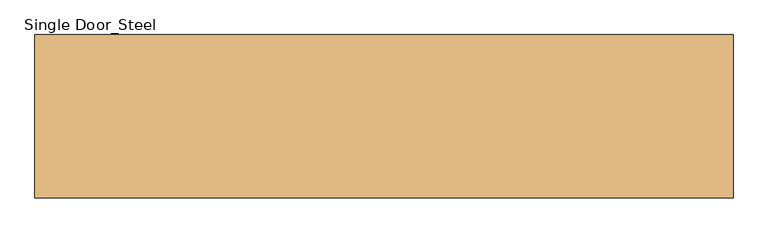
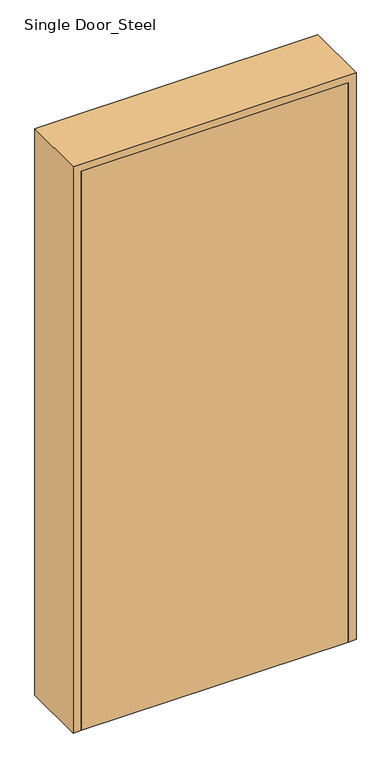
"""IFC4 building model written with IfcOpenShell, lengths in millimetres: door geometry, Single Door_Steel : H_DR_AR B12_Door_Single_W1100xH2280_FR 1.0H_FSD-1."""

from ifc_helpers import new_model, si_unit, origin, origin_with_axes, place, context, project, spatial, polyline, outline, extrude, faceted_brep, source, transform, mapped, element, save


def single_door_steel_8b0dfbf3(model_context):
    return source(origin(), model_context, "Body", "SolidModel", [
        extrude(outline(polyline([(505.0, -125.0), (-505.0, -125.0), (-505.0, -85.0), (505.0, -85.0), (505.0, -125.0)])), origin_with_axes(), (0.0, 0.0, 1.0), 2235.0),
        faceted_brep([(505.0, -125.0, 0.0), (505.0, -85.0, 0.0), (485.0, -85.0, 0.0), (485.0, 85.0, 0.0), (505.0, 85.0, 0.0), (505.0, 125.0, 0.0), (535.0, 125.0, 0.0), (535.0, -125.0, 0.0), (-505.0, -125.0, 0.0), (-535.0, -125.0, 0.0), (-535.0, 125.0, 0.0), (-505.0, 125.0, 0.0), (-505.0, 85.0, 0.0), (-485.0, 85.0, 0.0), (-485.0, -85.0, 0.0), (-505.0, -85.0, 0.0), (535.0, -125.0, 2265.0), (-535.0, -125.0, 2265.0), (-505.0, -125.0, 2235.0), (505.0, -125.0, 2235.0), (535.0, 125.0, 2265.0), (505.0, 125.0, 2235.0), (-505.0, 125.0, 2235.0), (-535.0, 125.0, 2265.0), (505.0, 85.0, 2235.0), (485.0, 85.0, 2215.0), (-485.0, 85.0, 2215.0), (-505.0, 85.0, 2235.0), (485.0, -85.0, 2215.0), (505.0, -85.0, 2235.0), (-505.0, -85.0, 2235.0), (-485.0, -85.0, 2215.0)], [[[0, 1, 2, 3, 4, 5, 6, 7]], [[8, 9, 10, 11, 12, 13, 14, 15]], [[7, 16, 17, 9, 8, 18, 19, 0]], [[6, 20, 16, 7]], [[5, 21, 22, 11, 10, 23, 20, 6]], [[4, 24, 21, 5]], [[3, 25, 26, 13, 12, 27, 24, 4]], [[2, 28, 25, 3]], [[1, 29, 30, 15, 14, 31, 28, 2]], [[0, 19, 29, 1]], [[18, 8, 15, 30]], [[23, 10, 9, 17]], [[27, 12, 11, 22]], [[31, 14, 13, 26]], [[20, 23, 17, 16]], [[24, 27, 22, 21]], [[28, 31, 26, 25]], [[19, 18, 30, 29]]]),
    ])


if __name__ == "__main__":
    model = new_model("IFC4")
    model_context = context("Model", 3, world=origin())
    ifc_project = project(units=[si_unit("LENGTHUNIT", "METRE", prefix="MILLI")], contexts=[model_context])
    site = spatial("IfcSite", under=ifc_project)
    building = spatial("IfcBuilding", under=site)
    placement = place(None, origin())
    single_door_steel_shape = single_door_steel_8b0dfbf3(model_context)
    element("IfcDoor", 1, ObjectType="Single Door_Steel : H_DR_AR B12_Door_Single_W1100xH2280_FR 1.0H_FSD-1", at=placement, inside=building, context=model_context, shape_type="MappedRepresentation", body=[
        mapped(single_door_steel_shape, transform((0.0, 0.0, 0.0), x_axis=(1.0, 0.0, 0.0), y_axis=(0.0, 1.0, 0.0), z_axis=(0.0, 0.0, 1.0))),
    ])
    save(model, "model.ifc")

# Revit data of these elements
# Type "Single Door_Steel : H_DR_AR B12_Door_Single_W1100xH2280_FR 1.0H_FSD-1"
#   Type Mark = "441"
#   Analytic Construction = "<None>"
#   프레임 투영 외부. = 25 mm
#   프레임 투영 내부. = 25 mm
#   프레임 폭 = 75 mm
#   Height = 2280 mm
#   Width = 1100 mm
#   Define Thermal Properties by = 1
#   문 패널 = none
#   문 프레임 = none
#   Function = (empty or 0)
#   Wall Closure = (empty or 0)
